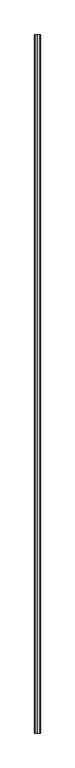
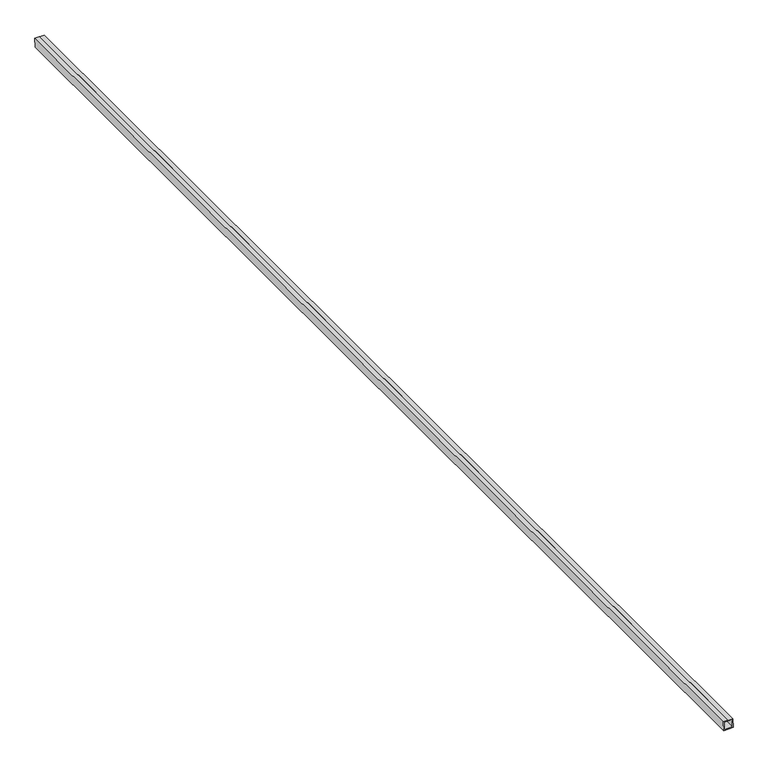
"""IFC4 building model written with IfcOpenShell, lengths in millimetres: proxy geometry, Inner panel:Inner panel:1:Inner panel:1 : Inner panel:Inner panel:300324:2:Inner panel:1:Inner panel:1 : Inner panel:Inner panel:300324:2 : Inner panel:Inner panel:1:Inner panel:1 : Inner panel:Inner panel:300324:300043:36 : Inner panel:Inner panel:1:Inner panel:1 : Inner panel:Inner panel:300324:2:Inner panel:1:Inner panel:1 : Inner panel:Inner panel:300324:2 : Inner panel:Inner panel:1:Inner panel:1 : Inner panel:Inner panel:300324:300043:308120."""

from ifc_helpers import new_model, si_unit, frame, origin, place, context, project, spatial, polyline, outline, extrude, source, transform, mapped, element, save


def generic_models_9bbaa720(model_context):
    return source(origin(), model_context, "Body", "SweptSolid", [
        extrude(outline(polyline([(3971.7309213, 560889.6434004), (3969.3517356, 560889.7425331), (3970.0126205, 560905.6037707), (3936.7040217, 560906.9916289), (3935.3161634, 560873.6830301), (3968.6247622, 560872.2951718), (3969.2856471, 560888.1564094), (3971.6648328, 560888.0572766), (3970.9048151, 560869.8168535), (3932.8378451, 560871.4029772), (3934.4239688, 560909.4699473), (3972.4909389, 560907.8838235), (3971.7309213, 560889.6434004)])), frame((0.0, -575657.416384, 0.0), z_axis=(0.0, 1.0, 0.0), x_axis=(0.0, 0.0, 1.0)), (0.0, 0.0, 1.0), 4876.8),
    ])


if __name__ == "__main__":
    model = new_model("IFC4")
    model_context = context("Model", 3, world=origin())
    ifc_project = project(units=[si_unit("LENGTHUNIT", "METRE", prefix="MILLI")], contexts=[model_context])
    site = spatial("IfcSite", under=ifc_project)
    building = spatial("IfcBuilding", under=site)
    placement = place(None, origin())
    generic_models_shape = generic_models_9bbaa720(model_context)
    element("IfcBuildingElementProxy", 1, Name="Inner panel:Inner panel:1:Inner panel:1 : Inner panel:Inner panel:300324:2:Inner panel:1:Inner panel:1 : Inner panel:Inner panel:300324:2 : Inner panel:Inner panel:1:Inner panel:1 : Inner panel:Inner panel:300324:300043:36 : Inner panel:Inner panel:1:Inner panel:1 : Inner panel:Inner panel:300324:2:Inner panel:1:Inner panel:1 : Inner panel:Inner panel:300324:2 : Inner panel:Inner panel:1:Inner panel:1 : Inner panel:Inner panel:300324:300043:308120", ObjectType="Inner panel:Inner panel:1:Inner panel:1 : Inner panel:Inner panel:300324:2:Inner panel:1:Inner panel:1 : Inner panel:Inner panel:300324:2 : Inner panel:Inner panel:1:Inner panel:1 : Inner panel:Inner panel:300324:300043:36 : Inner panel:Inner panel:1:Inner panel:1 : Inner panel:Inner panel:300324:2:Inner panel:1:Inner panel:1 : Inner panel:Inner panel:300324:2 : Inner panel:Inner panel:1:Inner panel:1 : Inner panel:Inner panel:300324:300043:308120", at=placement, inside=building, context=model_context, shape_type="MappedRepresentation", body=[
        mapped(generic_models_shape, transform((0.0, 0.0, 0.0), x_axis=(1.0, 0.0, 0.0), y_axis=(0.0, 1.0, 0.0), z_axis=(0.0, 0.0, 1.0))),
    ])
    save(model, "model.ifc")

# Revit data of these elements
# Type "Inner panel:Inner panel:1:Inner panel:1 : Inner panel:Inner panel:300324:2:Inner panel:1:Inner panel:1 : Inner panel:Inner panel:300324:2 : Inner panel:Inner panel:1:Inner panel:1 : Inner panel:Inner panel:300324:300043:36 : Inner panel:Inner panel:1:Inner panel:1 : Inner panel:Inner panel:300324:2:Inner panel:1:Inner panel:1 : Inner panel:Inner panel:300324:2 : Inner panel:Inner panel:1:Inner panel:1 : Inner panel:Inner panel:300324:300043:308120"
#   NameOverride = "Inner panel:Inner panel:1:Inner panel:1 : Inner panel:Inner panel:300324:2:Inner panel:1:Inner panel:1 : Inner panel:Inner panel:300324:2 : Inner panel:Inner panel:1:Inner panel:1 : Inner panel:Inner panel:300324:300043:308120"
#   ObjectTypeOverride = "Inner panel:1:Inner panel:1 : Inner panel:Inner panel:300324:2 : Inner panel:Inner panel:1:Inner panel:1 : Inner panel:Inner panel:300324:300043"
#   Reference = "Inner panel"
#   Tag = "308120"
# Element 1 (IfcBuildingElementProxy, "Inner panel:Inner panel:1:Inner panel:1 : Inner panel:Inner panel:300324:2:Inner panel:1:Inner panel:1 : Inner panel:Inner panel:300324:2 : Inner panel:Inner panel:1:Inner panel:1 : Inner panel:Inner panel:300324:300043:36 : Inner panel:Inner panel:1:Inner panel:1 : Inner panel:Inner panel:300324:2:Inner panel:1:Inner panel:1 : Inner panel:Inner panel:300324:2 : Inner panel:Inner panel:1:Inner panel:1 : Inner panel:Inner panel:300324:300043:308120")
#   Materials on its faces: "1 1/2\" X 1 1/2\" x 1/8\" ALUM. TUBE (6061-T6) - (2) #16 WOOD SCREWS WITH 2.5\" EMBED AT EACH GLULAM - (1) SCREW AT ENDS"
# Materials
#   "1 1/2\" X 1 1/2\" x 1/8\" ALUM. TUBE (6061-T6) - (2) #16 WOOD SCREWS WITH 2.5\" EMBED AT EACH GLULAM - (1) SCREW AT ENDS": class "Unassigned", colour RGB 202 201 200, transparency 0, Cost = 0
